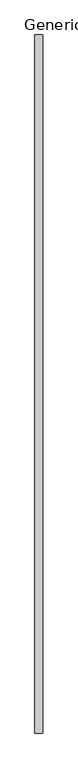
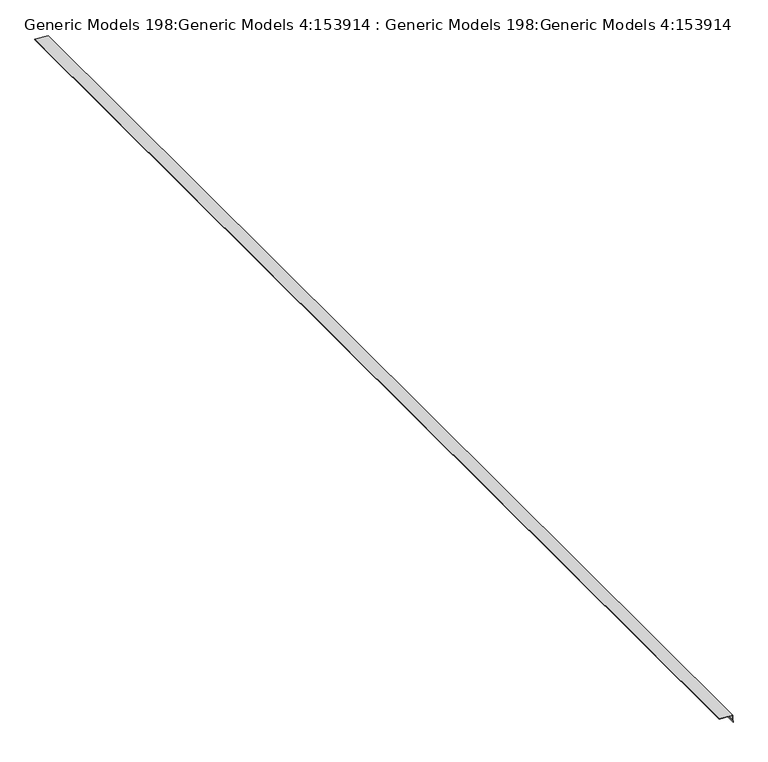
"""IFC4 building model written with IfcOpenShell, lengths in millimetres: proxy geometry, Generic Models 198:Generic Models 4:153914 : Generic Models 198:Generic Models 4:153914."""

from ifc_helpers import new_model, si_unit, frame, origin, place, context, project, spatial, polyline, outline, extrude, source, transform, mapped, element, save


def generic_models_198_generic_models_4_153914_generic_models_898556cd(model_context):
    return source(origin(), model_context, "Body", "SweptSolid", [
        extrude(outline(polyline([(3561.7053156, -8204.2049913), (3554.5733751, -8201.6091772), (3535.5394151, -8201.6091772), (3535.5394151, -8200.8154272), (3554.7133346, -8200.8154272), (3561.8452752, -8203.4112413), (3627.9884476, -8203.4112413), (3634.5874421, -8361.7871085), (3633.7943802, -8361.8201527), (3627.2270818, -8204.2049913), (3561.7053156, -8204.2049913)])), frame((0.0, -6674.7974793, 0.0), z_axis=(0.0, 1.0, 0.0), x_axis=(0.0, 0.0, 1.0)), (0.0, 0.0, 1.0), 13919.2),
    ])


if __name__ == "__main__":
    model = new_model("IFC4")
    model_context = context("Model", 3, world=origin())
    ifc_project = project(units=[si_unit("LENGTHUNIT", "METRE", prefix="MILLI")], contexts=[model_context])
    site = spatial("IfcSite", under=ifc_project)
    building = spatial("IfcBuilding", under=site)
    placement = place(None, origin())
    generic_models_198_generic_models_4_153914_generic_models_shape = generic_models_198_generic_models_4_153914_generic_models_898556cd(model_context)
    element("IfcBuildingElementProxy", 1, Name="Generic Models 198:Generic Models 4:153914 : Generic Models 198:Generic Models 4:153914", ObjectType="Generic Models 198:Generic Models 4:153914 : Generic Models 198:Generic Models 4:153914", at=placement, inside=building, context=model_context, shape_type="MappedRepresentation", body=[
        mapped(generic_models_198_generic_models_4_153914_generic_models_shape, transform((0.0, 0.0, 0.0), x_axis=(1.0, 0.0, 0.0), y_axis=(0.0, 1.0, 0.0), z_axis=(0.0, 0.0, 1.0))),
    ])
    save(model, "model.ifc")

# Revit data of these elements
# Type "Generic Models 198:Generic Models 4:153914 : Generic Models 198:Generic Models 4:153914"
#   NameOverride = "Generic Models 198:Generic Models 4:153914"
#   ObjectTypeOverride = "Generic Models 198:Generic Models 4"
#   Reference = "Generic Models 4"
#   Category = "Generic Models"
#   Tag = "153914"
# Element 1 (IfcBuildingElementProxy, "Generic Models 198:Generic Models 4:153914 : Generic Models 198:Generic Models 4:153914")
#   Materials on its faces: "_(2) LAYERS NO. 30 ASTM D226 ASPHALT SATURATED ORGANIC FELT 997"
# Materials
#   "_(2) LAYERS NO. 30 ASTM D226 ASPHALT SATURATED ORGANIC FELT 997": class "Unassigned", colour RGB 67 154 161, transparency 0
